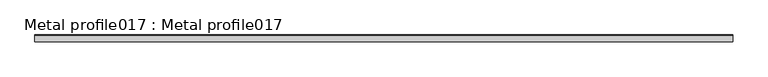
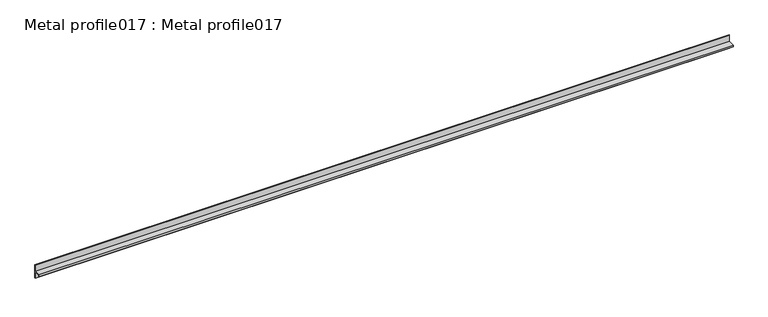
"""IFC4 building model written with IfcOpenShell, lengths in millimetres: proxy geometry, Metal profile017 : Metal profile017."""

from ifc_helpers import new_model, si_unit, frame, origin, place, context, project, spatial, polyline, outline, extrude, source, transform, mapped, element, save


def metal_profile017_metal_profile017_bf22f2e0(model_context):
    return source(origin(), model_context, "Body", "SweptSolid", [
        extrude(outline(polyline([(-4680.7217972, 38395.4682813), (-4680.7217972, 38391.9884812), (-4681.9917972, 38391.9884812), (-4681.9917972, 38396.7382812), (-4663.7578493, 38396.7382812), (-4663.7578493, 38415.7882812), (-4662.4878493, 38415.7882812), (-4662.4878493, 38376.4182812), (-4663.7578493, 38376.4182812), (-4663.7578493, 38395.4682813), (-4680.7217972, 38395.4682813)])), frame((12383.0178845, 0.0, 0.0), z_axis=(1.0, 0.0, 0.0), x_axis=(0.0, 1.0, 0.0)), (0.0, 0.0, 1.0), 2000.0),
    ])


if __name__ == "__main__":
    model = new_model("IFC4")
    model_context = context("Model", 3, world=origin())
    ifc_project = project(units=[si_unit("LENGTHUNIT", "METRE", prefix="MILLI")], contexts=[model_context])
    site = spatial("IfcSite", under=ifc_project)
    building = spatial("IfcBuilding", under=site)
    placement = place(None, origin())
    metal_profile017_metal_profile017_shape = metal_profile017_metal_profile017_bf22f2e0(model_context)
    element("IfcBuildingElementProxy", 1, Name="Metal profile017 : Metal profile017", ObjectType="Metal profile017 : Metal profile017", at=placement, inside=building, context=model_context, shape_type="MappedRepresentation", body=[
        mapped(metal_profile017_metal_profile017_shape, transform((0.0, 0.0, 0.0), x_axis=(1.0, 0.0, 0.0), y_axis=(0.0, 1.0, 0.0), z_axis=(0.0, 0.0, 1.0))),
    ])
    save(model, "model.ifc")

# Revit data of these elements
# Type "Metal profile017 : Metal profile017"
#   NameOverride = "Metal profile017"
# Element 1 (IfcBuildingElementProxy, "Metal profile017 : Metal profile017")
#   Materials on its faces: "16 GA. COPPER VENTED T REVEAL BEAD"
# Materials
#   "16 GA. COPPER VENTED T REVEAL BEAD": class "Unassigned", colour RGB 255 227 10, transparency 0
